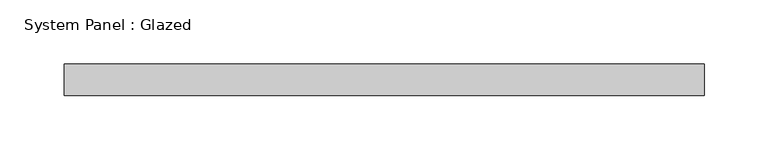
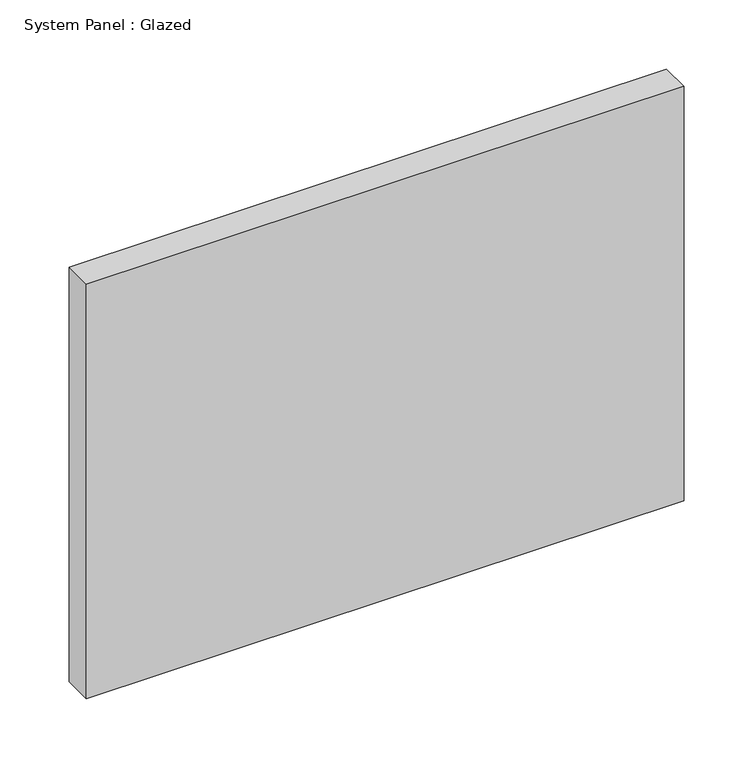
"""IFC4 building model written with IfcOpenShell, lengths in millimetres: plate geometry, System Panel : Glazed."""

from ifc_helpers import new_model, si_unit, origin, origin_with_axes, place, context, project, spatial, polyline, outline, extrude, source, transform, mapped, element, save


def system_panel_glazed_8d9a0772(model_context):
    return source(origin(), model_context, "Body", "SweptSolid", [
        extrude(outline(polyline([(250.0, 24.5), (-250.0, 24.5), (-250.0, 49.5), (250.0, 49.5), (250.0, 24.5)])), origin_with_axes(), (0.0, 0.0, 1.0), 366.6666667),
    ])


if __name__ == "__main__":
    model = new_model("IFC4")
    model_context = context("Model", 3, world=origin())
    ifc_project = project(units=[si_unit("LENGTHUNIT", "METRE", prefix="MILLI")], contexts=[model_context])
    site = spatial("IfcSite", under=ifc_project)
    building = spatial("IfcBuilding", under=site)
    placement = place(None, origin())
    system_panel_glazed_shape = system_panel_glazed_8d9a0772(model_context)
    element("IfcPlate", 1, ObjectType="System Panel : Glazed", at=placement, inside=building, context=model_context, shape_type="MappedRepresentation", body=[
        mapped(system_panel_glazed_shape, transform((0.0, 0.0, 0.0), x_axis=(1.0, 0.0, 0.0), y_axis=(0.0, 1.0, 0.0), z_axis=(0.0, 0.0, 1.0))),
    ])
    save(model, "model.ifc")

# Revit data of these elements
# Element 1 (IfcPlate, "System Panel : Glazed")
#   Materials on its faces: "Glass"
# Materials
#   "Glass": class "Glass", colour RGB 218 227 224, transparency 0.85, Description = "Soda Lime Glass", Cost = 0
